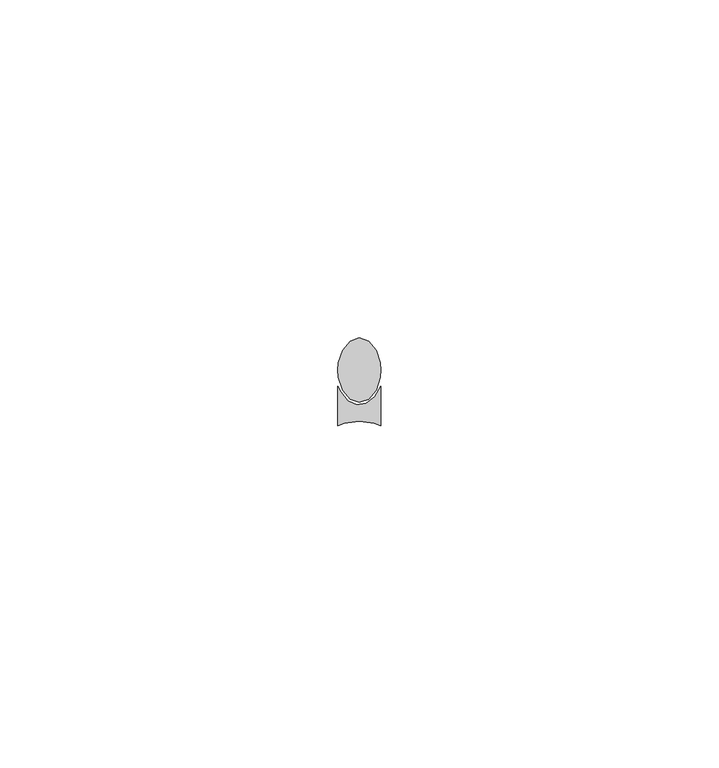
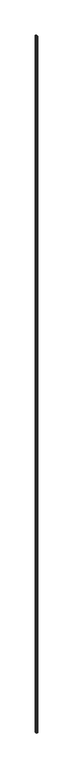
"""IFC4 building model written with IfcOpenShell, lengths in millimetres: proxy geometry, Generic Models 11:Generic Models 1:306267:Generic Models 1:306267 : Generic Models 11:Generic Models 1:306267:300405:Generic Models 1:306267:Generic Models 1:306267 : Generic Models 11:Generic Models 1:306267:300405 : Generic Models 11:Generic Models 1:306267:Generic Models 1:306267 : Generic Models 11:Generic Models 1:306267:300405:1 : Generic Models 11:Generic Models 1:306267:Generic Models 1:306267 : Generic Models 11:Generic Models 1:306267:300405:Generic Models 1:306267:Generic Models 1:306267 : Generic Models 11:Generic Models 1:306267:300405 : Generic Models 11:Generic Models 1:306267:Generic Models 1:306267 : Generic Models 11:Generic Models 1:306267:300405:300182."""

from ifc_helpers import new_model, si_unit, origin, origin_with_axes, place, context, project, spatial, polyline, outline, extrude, source, transform, mapped, element, save


def generic_models_188393ea(model_context):
    return source(origin(), model_context, "Body", "SweptSolid", [
        extrude(outline(polyline([(593733.5341431, -579092.0005286), (593732.429409, -579090.6790346), (593731.8163278, -579088.7694203), (593731.7367239, -579087.7096644), (593731.8163278, -579086.6499084), (593732.429409, -579084.7402942), (593733.5341431, -579083.4188002), (593734.9117239, -579082.9471644), (593736.2893048, -579083.4188002), (593737.3940389, -579084.7402942), (593738.0071201, -579086.6499084), (593738.0867239, -579087.7096644), (593738.0071201, -579088.7694203), (593737.3940389, -579090.6790346), (593736.2893048, -579092.0005286), (593734.9117239, -579092.4721644), (593733.5341431, -579092.0005286)])), origin_with_axes(), (0.0, 0.0, 1.0), 3702.05),
        extrude(outline(polyline([(593737.1209607, -579095.5639755), (593734.9117239, -579095.2502894), (593732.7024872, -579095.5639755), (593731.7367239, -579095.9413841), (593731.7367239, -579090.073292), (593732.1230415, -579090.9335729), (593733.206527, -579092.2431481), (593734.5567747, -579092.8435016), (593735.962551, -579092.6407137), (593737.2039351, -579091.6665087), (593738.0867239, -579090.073292), (593738.0867239, -579095.9413841), (593737.1209607, -579095.5639755)])), origin_with_axes(), (0.0, 0.0, 1.0), 3702.05),
    ])


if __name__ == "__main__":
    model = new_model("IFC4")
    model_context = context("Model", 3, world=origin())
    ifc_project = project(units=[si_unit("LENGTHUNIT", "METRE", prefix="MILLI")], contexts=[model_context])
    site = spatial("IfcSite", under=ifc_project)
    building = spatial("IfcBuilding", under=site)
    placement = place(None, origin())
    generic_models_shape = generic_models_188393ea(model_context)
    element("IfcBuildingElementProxy", 1, Name="Generic Models 11:Generic Models 1:306267:Generic Models 1:306267 : Generic Models 11:Generic Models 1:306267:300405:Generic Models 1:306267:Generic Models 1:306267 : Generic Models 11:Generic Models 1:306267:300405 : Generic Models 11:Generic Models 1:306267:Generic Models 1:306267 : Generic Models 11:Generic Models 1:306267:300405:1 : Generic Models 11:Generic Models 1:306267:Generic Models 1:306267 : Generic Models 11:Generic Models 1:306267:300405:Generic Models 1:306267:Generic Models 1:306267 : Generic Models 11:Generic Models 1:306267:300405 : Generic Models 11:Generic Models 1:306267:Generic Models 1:306267 : Generic Models 11:Generic Models 1:306267:300405:300182", ObjectType="Generic Models 11:Generic Models 1:306267:Generic Models 1:306267 : Generic Models 11:Generic Models 1:306267:300405:Generic Models 1:306267:Generic Models 1:306267 : Generic Models 11:Generic Models 1:306267:300405 : Generic Models 11:Generic Models 1:306267:Generic Models 1:306267 : Generic Models 11:Generic Models 1:306267:300405:1 : Generic Models 11:Generic Models 1:306267:Generic Models 1:306267 : Generic Models 11:Generic Models 1:306267:300405:Generic Models 1:306267:Generic Models 1:306267 : Generic Models 11:Generic Models 1:306267:300405 : Generic Models 11:Generic Models 1:306267:Generic Models 1:306267 : Generic Models 11:Generic Models 1:306267:300405:300182", at=placement, inside=building, context=model_context, shape_type="MappedRepresentation", body=[
        mapped(generic_models_shape, transform((0.0, 0.0, 0.0), x_axis=(1.0, 0.0, 0.0), y_axis=(0.0, 1.0, 0.0), z_axis=(0.0, 0.0, 1.0))),
    ])
    save(model, "model.ifc")

# Revit data of these elements
# Type "Generic Models 11:Generic Models 1:306267:Generic Models 1:306267 : Generic Models 11:Generic Models 1:306267:300405:Generic Models 1:306267:Generic Models 1:306267 : Generic Models 11:Generic Models 1:306267:300405 : Generic Models 11:Generic Models 1:306267:Generic Models 1:306267 : Generic Models 11:Generic Models 1:306267:300405:1 : Generic Models 11:Generic Models 1:306267:Generic Models 1:306267 : Generic Models 11:Generic Models 1:306267:300405:Generic Models 1:306267:Generic Models 1:306267 : Generic Models 11:Generic Models 1:306267:300405 : Generic Models 11:Generic Models 1:306267:Generic Models 1:306267 : Generic Models 11:Generic Models 1:306267:300405:300182"
#   NameOverride = "Generic Models 11:Generic Models 1:306267:Generic Models 1:306267 : Generic Models 11:Generic Models 1:306267:300405:Generic Models 1:306267:Generic Models 1:306267 : Generic Models 11:Generic Models 1:306267:300405 : Generic Models 11:Generic Models 1:306267:Generic Models 1:306267 : Generic Models 11:Generic Models 1:306267:300405:300182"
#   ObjectTypeOverride = "Generic Models 1:306267:Generic Models 1:306267 : Generic Models 11:Generic Models 1:306267:300405 : Generic Models 11:Generic Models 1:306267:Generic Models 1:306267 : Generic Models 11:Generic Models 1:306267:300405"
#   Reference = "Generic Models 1"
#   Tag = "300182"
# Element 1 (IfcBuildingElementProxy, "Generic Models 11:Generic Models 1:306267:Generic Models 1:306267 : Generic Models 11:Generic Models 1:306267:300405:Generic Models 1:306267:Generic Models 1:306267 : Generic Models 11:Generic Models 1:306267:300405 : Generic Models 11:Generic Models 1:306267:Generic Models 1:306267 : Generic Models 11:Generic Models 1:306267:300405:1 : Generic Models 11:Generic Models 1:306267:Generic Models 1:306267 : Generic Models 11:Generic Models 1:306267:300405:Generic Models 1:306267:Generic Models 1:306267 : Generic Models 11:Generic Models 1:306267:300405 : Generic Models 11:Generic Models 1:306267:Generic Models 1:306267 : Generic Models 11:Generic Models 1:306267:300405:300182")
#   Materials on its faces: "SEALANT & BACKER ROD, IF NECESSARY"
# Materials
#   "SEALANT & BACKER ROD, IF NECESSARY": class "Unassigned", colour RGB 120 120 120, transparency 0, Cost = 0
